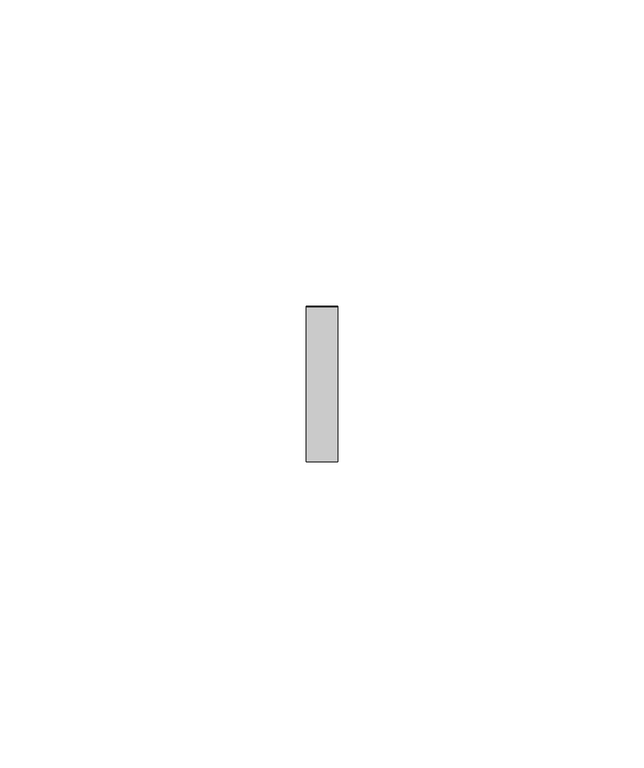
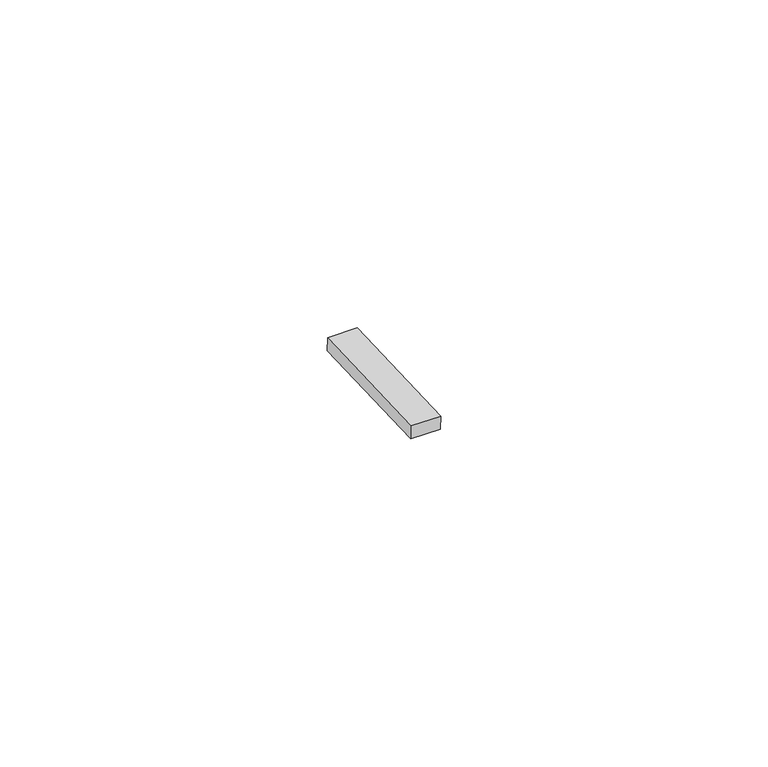
"""IFC4 building model written with IfcOpenShell, lengths in millimetres: proxy geometry, Inner panel:Inner panel:1:Inner panel:1 : Inner panel:Inner panel:300324:2:Inner panel:1:Inner panel:1 : Inner panel:Inner panel:300324:2 : Inner panel:Inner panel:1:Inner panel:1 : Inner panel:Inner panel:300324:300043:131 : Inner panel:Inner panel:1:Inner panel:1 : Inner panel:Inner panel:300324:2:Inner panel:1:Inner panel:1 : Inner panel:Inner panel:300324:2 : Inner panel:Inner panel:1:Inner panel:1 : Inner panel:Inner panel:300324:300043:308120."""

import ifcopenshell
import ifcopenshell.guid

model = None  # the IFC model being written
_history = None  # IfcOwnerHistory: only IFC2X3 demands one
_inside = {}  # id of a spatial element -> (the spatial element, [elements in it])
_under = {}  # id of a project, library or spatial element -> (it, [spatial elements below it])
_declared = {}  # id of a project -> (the project, [libraries it declares])
_typed = {}  # id of a type object -> (the type object, [elements of that type])
_made_of = {}  # id of a material, layer set ... -> (it, [elements and type objects made of it])


def new_model(schema):
    """Start an empty IFC model of exactly this schema.

    Asked for "IFC4X3", IfcOpenShell would pick the latest addendum, in which some entities
    have other attributes; the version numbers below select the first issue.
    IFC2X3 requires an IfcOwnerHistory on every rooted entity: one is made here for all.
    """
    global model, _history
    if schema == "IFC4X3":
        model = ifcopenshell.file(schema_version=(4, 3, 0, 0))
    else:
        model = ifcopenshell.file(schema=schema)
    _inside.clear()
    _under.clear()
    _declared.clear()
    _typed.clear()
    _made_of.clear()
    _history = None
    if model.schema == "IFC2X3":
        org = make("IfcOrganization", Name="unknown")
        user = make(
            "IfcPersonAndOrganization",
            ThePerson=make("IfcPerson", FamilyName="unknown"),
            TheOrganization=org,
        )
        app = make(
            "IfcApplication",
            ApplicationDeveloper=org,
            Version="unknown",
            ApplicationFullName="unknown",
            ApplicationIdentifier="unknown",
        )
        _history = make(
            "IfcOwnerHistory",
            OwningUser=user,
            OwningApplication=app,
            ChangeAction="ADDED",
            CreationDate=0,
        )
    return model


def make(cls, **values):
    """One entity of the class cls with the attributes given. An attribute that is None is left unset."""
    return model.create_entity(
        cls, **{name: value for name, value in values.items() if value is not None}
    )


def rooted(cls, **values):
    """An entity with a GlobalId (a new one), such as an element, a storey or a relation."""
    return make(cls, GlobalId=ifcopenshell.guid.new(), OwnerHistory=_history, **values)


def si_unit(unit_type, name, prefix=None):
    """IfcSIUnit, for example si_unit("LENGTHUNIT", "METRE", prefix="MILLI")."""
    return make("IfcSIUnit", UnitType=unit_type, Prefix=prefix, Name=name)


def assignment(units):
    """IfcUnitAssignment: the units of a project."""
    return None if units is None else make("IfcUnitAssignment", Units=units)


def point(xyz):
    """IfcCartesianPoint."""
    return None if xyz is None else make("IfcCartesianPoint", Coordinates=xyz)


def direction(xyz):
    """IfcDirection."""
    return None if xyz is None else make("IfcDirection", DirectionRatios=xyz)


def frame(location, z_axis=None, x_axis=None):
    """IfcAxis2Placement3D, a coordinate frame: its origin and axes. An axis left out is left unset."""
    return make(
        "IfcAxis2Placement3D",
        Location=point(location),
        Axis=direction(z_axis),
        RefDirection=direction(x_axis),
    )


def origin():
    """The frame at (0, 0, 0) with its axes left unset."""
    return frame((0.0, 0.0, 0.0))


def place(relative_to, where):
    """IfcLocalPlacement: puts the frame where relative to a parent placement (None: the world)."""
    return make(
        "IfcLocalPlacement", PlacementRelTo=relative_to, RelativePlacement=where
    )


def context(
    kind, dimensions, precision=None, world=None, true_north=None, identifier=None
):
    """IfcGeometricRepresentationContext, for example the 3D "Model" context."""
    return make(
        "IfcGeometricRepresentationContext",
        ContextIdentifier=identifier,
        ContextType=kind,
        CoordinateSpaceDimension=dimensions,
        Precision=precision,
        WorldCoordinateSystem=world,
        TrueNorth=true_north,
    )


def project(units=None, contexts=None):
    """IfcProject with its units and contexts."""
    return rooted(
        "IfcProject",
        Name="project",
        RepresentationContexts=contexts,
        UnitsInContext=assignment(units),
    )


def spatial(cls, under=None, at=None, **own):
    """A site, building, storey or space (cls), placed at a placement, below another one or the project."""
    s = rooted(cls, ObjectPlacement=at, **own)
    if under is not None:
        _under.setdefault(under.id(), (under, []))[1].append(s)
    return s


def polyline(points):
    """IfcPolyline through the points."""
    return make("IfcPolyline", Points=[point(p) for p in points])


def outline(outer, holes=None, kind="AREA"):
    """IfcArbitraryClosedProfileDef: a profile drawn as a closed curve; with holes, ...WithVoids."""
    if holes is None:
        return make("IfcArbitraryClosedProfileDef", ProfileType=kind, OuterCurve=outer)
    return make(
        "IfcArbitraryProfileDefWithVoids",
        ProfileType=kind,
        OuterCurve=outer,
        InnerCurves=holes,
    )


def extrude(swept, where, along, depth):
    """IfcExtrudedAreaSolid: the profile swept, set in the frame where, extruded along a direction by depth."""
    return make(
        "IfcExtrudedAreaSolid",
        SweptArea=swept,
        Position=where,
        ExtrudedDirection=direction(along),
        Depth=depth,
    )


def shape(context_of_items, identifier, shape_type, items):
    """IfcShapeRepresentation: the items that make up one representation, for example the "Body"."""
    return make(
        "IfcShapeRepresentation",
        ContextOfItems=context_of_items,
        RepresentationIdentifier=identifier,
        RepresentationType=shape_type,
        Items=items,
    )


def source(mapping_origin, context_of_items, identifier, shape_type, items):
    """IfcRepresentationMap: a shape defined once, which mapped items show again and again."""
    return make(
        "IfcRepresentationMap",
        MappingOrigin=mapping_origin,
        MappedRepresentation=shape(context_of_items, identifier, shape_type, items),
    )


def transform(
    local_origin,
    x_axis=None,
    y_axis=None,
    z_axis=None,
    scale=None,
    scale2=None,
    scale3=None,
    uniform=True,
):
    """IfcCartesianTransformationOperator3D, or its non-uniform kind. x_axis, y_axis, z_axis: its Axis1, 2, 3."""
    if uniform:
        return make(
            "IfcCartesianTransformationOperator3D",
            Axis1=direction(x_axis),
            Axis2=direction(y_axis),
            LocalOrigin=point(local_origin),
            Scale=scale,
            Axis3=direction(z_axis),
        )
    return make(
        "IfcCartesianTransformationOperator3DnonUniform",
        Axis1=direction(x_axis),
        Axis2=direction(y_axis),
        LocalOrigin=point(local_origin),
        Scale=scale,
        Axis3=direction(z_axis),
        Scale2=scale2,
        Scale3=scale3,
    )


def mapped(mapping_source, mapping_target):
    """IfcMappedItem: shows the shape of a source again, moved by a transform."""
    return make(
        "IfcMappedItem", MappingSource=mapping_source, MappingTarget=mapping_target
    )


def made_of(thing, what):
    """Note that an element or type object is made of a material, layer set ...; save() writes the relation."""
    if what is not None:
        _made_of.setdefault(what.id(), (what, []))[1].append(thing)
    return thing


def element(
    cls,
    number,
    at=None,
    inside=None,
    cuts=None,
    type_object=None,
    material=None,
    context=None,
    identifier="Body",
    shape_type=None,
    held_by="IfcProductDefinitionShape",
    body=None,
    shapes=None,
    **own,
):
    """One element of the class cls, such as IfcWall. Its Tag is "e" and its number.

    at: its placement. inside: the storey or other place that contains it. cuts: it is an
    opening in that element (IfcRelVoidsElement). A single representation is given by context,
    identifier, shape_type and body (its items); several are given by shapes. held_by: the class
    of the entity that holds the representations. save() writes the other relations.
    """
    e = rooted(cls, Tag="e%d" % number, ObjectPlacement=at, **own)
    if body is not None:
        shapes = [shape(context, identifier, shape_type, body)]
    if shapes is not None:
        e.Representation = make(held_by, Representations=shapes)
    if inside is not None:
        _inside.setdefault(inside.id(), (inside, []))[1].append(e)
    if cuts is not None:
        rooted(
            "IfcRelVoidsElement", RelatingBuildingElement=cuts, RelatedOpeningElement=e
        )
    if type_object is not None:
        _typed.setdefault(type_object.id(), (type_object, []))[1].append(e)
    return made_of(e, material)


def aggregate(whole, parts):
    """IfcRelAggregates: a whole, such as a stair, and the parts it consists of."""
    return rooted("IfcRelAggregates", RelatingObject=whole, RelatedObjects=parts)


def save(model, path):
    """Write the relations noted so far, then the file.

    IfcRelAggregates (storeys below a building ...), IfcRelContainedInSpatialStructure (elements
    in a storey), IfcRelDefinesByType, IfcRelAssociatesMaterial and IfcRelDeclares: one each for
    every whole, place, type object, material and project.
    """
    for whole, parts in _under.values():
        aggregate(whole, parts)
    for where, things in _inside.values():
        rooted(
            "IfcRelContainedInSpatialStructure",
            RelatedElements=things,
            RelatingStructure=where,
        )
    for kind, things in _typed.values():
        rooted("IfcRelDefinesByType", RelatedObjects=things, RelatingType=kind)
    for what, things in _made_of.values():
        rooted("IfcRelAssociatesMaterial", RelatedObjects=things, RelatingMaterial=what)
    for by, libraries in _declared.values():
        rooted("IfcRelDeclares", RelatingContext=by, RelatedDefinitions=libraries)
    model.write(path)


def generic_models_c81a9b6a(model_context):
    return source(origin(), model_context, "Body", "SweptSolid", [
        extrude(outline(polyline([(0.0, -25.4), (0.0, 0.0), (5.2138089, 0.0), (5.2138089, -25.4), (0.0, -25.4)])), frame((592717.395117, -576574.3073926, 4050.9976844), z_axis=(0.0, -0.041630544712223896, 0.9991330730923502), x_axis=(-1.0, 0.0, 0.0)), (0.0, 0.0, 1.0), 2.4763745),
    ])


if __name__ == "__main__":
    model = new_model("IFC4")
    model_context = context("Model", 3, world=origin())
    ifc_project = project(units=[si_unit("LENGTHUNIT", "METRE", prefix="MILLI")], contexts=[model_context])
    site = spatial("IfcSite", under=ifc_project)
    building = spatial("IfcBuilding", under=site)
    placement = place(None, origin())
    generic_models_shape = generic_models_c81a9b6a(model_context)
    element("IfcBuildingElementProxy", 1, Name="Inner panel:Inner panel:1:Inner panel:1 : Inner panel:Inner panel:300324:2:Inner panel:1:Inner panel:1 : Inner panel:Inner panel:300324:2 : Inner panel:Inner panel:1:Inner panel:1 : Inner panel:Inner panel:300324:300043:131 : Inner panel:Inner panel:1:Inner panel:1 : Inner panel:Inner panel:300324:2:Inner panel:1:Inner panel:1 : Inner panel:Inner panel:300324:2 : Inner panel:Inner panel:1:Inner panel:1 : Inner panel:Inner panel:300324:300043:308120", ObjectType="Inner panel:Inner panel:1:Inner panel:1 : Inner panel:Inner panel:300324:2:Inner panel:1:Inner panel:1 : Inner panel:Inner panel:300324:2 : Inner panel:Inner panel:1:Inner panel:1 : Inner panel:Inner panel:300324:300043:131 : Inner panel:Inner panel:1:Inner panel:1 : Inner panel:Inner panel:300324:2:Inner panel:1:Inner panel:1 : Inner panel:Inner panel:300324:2 : Inner panel:Inner panel:1:Inner panel:1 : Inner panel:Inner panel:300324:300043:308120", at=placement, inside=building, context=model_context, shape_type="MappedRepresentation", body=[
        mapped(generic_models_shape, transform((0.0, 0.0, 0.0), x_axis=(1.0, 0.0, 0.0), y_axis=(0.0, 1.0, 0.0), z_axis=(0.0, 0.0, 1.0))),
    ])
    save(model, "model.ifc")

# Revit data of these elements
# Type "Inner panel:Inner panel:1:Inner panel:1 : Inner panel:Inner panel:300324:2:Inner panel:1:Inner panel:1 : Inner panel:Inner panel:300324:2 : Inner panel:Inner panel:1:Inner panel:1 : Inner panel:Inner panel:300324:300043:131 : Inner panel:Inner panel:1:Inner panel:1 : Inner panel:Inner panel:300324:2:Inner panel:1:Inner panel:1 : Inner panel:Inner panel:300324:2 : Inner panel:Inner panel:1:Inner panel:1 : Inner panel:Inner panel:300324:300043:308120"
#   NameOverride = "Inner panel:Inner panel:1:Inner panel:1 : Inner panel:Inner panel:300324:2:Inner panel:1:Inner panel:1 : Inner panel:Inner panel:300324:2 : Inner panel:Inner panel:1:Inner panel:1 : Inner panel:Inner panel:300324:300043:308120"
#   ObjectTypeOverride = "Inner panel:1:Inner panel:1 : Inner panel:Inner panel:300324:2 : Inner panel:Inner panel:1:Inner panel:1 : Inner panel:Inner panel:300324:300043"
#   Reference = "Inner panel"
#   Tag = "308120"
# Element 1 (IfcBuildingElementProxy, "Inner panel:Inner panel:1:Inner panel:1 : Inner panel:Inner panel:300324:2:Inner panel:1:Inner panel:1 : Inner panel:Inner panel:300324:2 : Inner panel:Inner panel:1:Inner panel:1 : Inner panel:Inner panel:300324:300043:131 : Inner panel:Inner panel:1:Inner panel:1 : Inner panel:Inner panel:300324:2:Inner panel:1:Inner panel:1 : Inner panel:Inner panel:300324:2 : Inner panel:Inner panel:1:Inner panel:1 : Inner panel:Inner panel:300324:300043:308120")
#   Materials on its faces: "AT CLIP - 1\" WIDE NON ABSORBENT, WEATHER-RESISTANT NEOPRENE/EPDM/SBR FOAM"
# Materials
#   "AT CLIP - 1\" WIDE NON ABSORBENT, WEATHER-RESISTANT NEOPRENE/EPDM/SBR FOAM": class "Generic", colour RGB 85 85 85, transparency 0, Cost = 0
